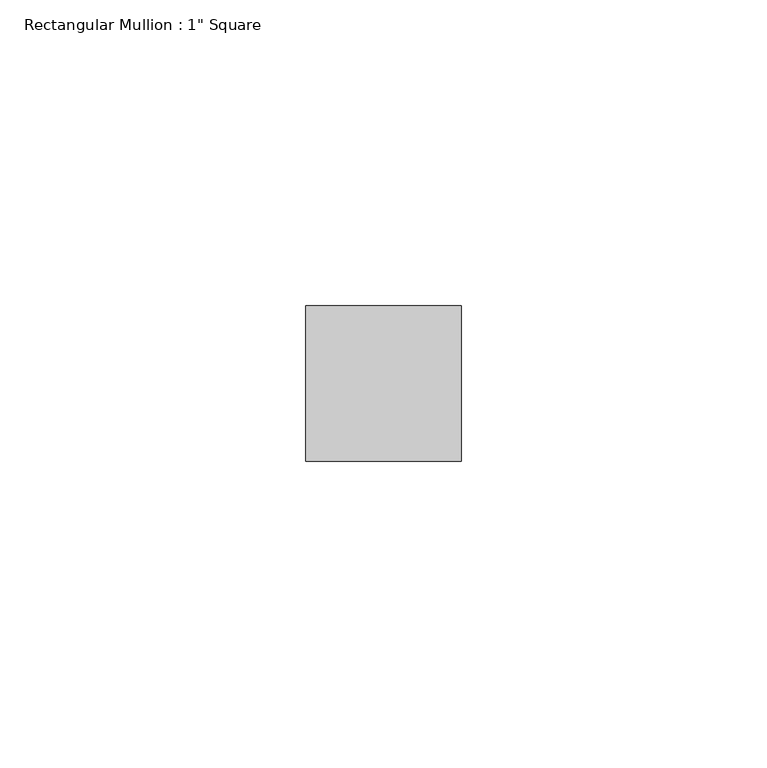
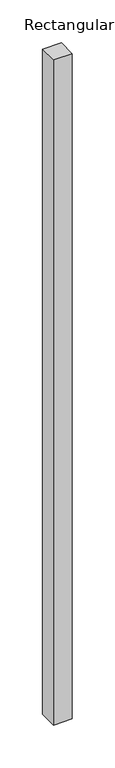
"""IFC4 building model written with IfcOpenShell, lengths in millimetres: member geometry."""

import ifcopenshell
import ifcopenshell.guid

model = None  # the IFC model being written
_history = None  # IfcOwnerHistory: only IFC2X3 demands one
_inside = {}  # id of a spatial element -> (the spatial element, [elements in it])
_under = {}  # id of a project, library or spatial element -> (it, [spatial elements below it])
_declared = {}  # id of a project -> (the project, [libraries it declares])
_typed = {}  # id of a type object -> (the type object, [elements of that type])
_made_of = {}  # id of a material, layer set ... -> (it, [elements and type objects made of it])


def new_model(schema):
    """Start an empty IFC model of exactly this schema.

    Asked for "IFC4X3", IfcOpenShell would pick the latest addendum, in which some entities
    have other attributes; the version numbers below select the first issue.
    IFC2X3 requires an IfcOwnerHistory on every rooted entity: one is made here for all.
    """
    global model, _history
    if schema == "IFC4X3":
        model = ifcopenshell.file(schema_version=(4, 3, 0, 0))
    else:
        model = ifcopenshell.file(schema=schema)
    _inside.clear()
    _under.clear()
    _declared.clear()
    _typed.clear()
    _made_of.clear()
    _history = None
    if model.schema == "IFC2X3":
        org = make("IfcOrganization", Name="unknown")
        user = make(
            "IfcPersonAndOrganization",
            ThePerson=make("IfcPerson", FamilyName="unknown"),
            TheOrganization=org,
        )
        app = make(
            "IfcApplication",
            ApplicationDeveloper=org,
            Version="unknown",
            ApplicationFullName="unknown",
            ApplicationIdentifier="unknown",
        )
        _history = make(
            "IfcOwnerHistory",
            OwningUser=user,
            OwningApplication=app,
            ChangeAction="ADDED",
            CreationDate=0,
        )
    return model


def make(cls, **values):
    """One entity of the class cls with the attributes given. An attribute that is None is left unset."""
    return model.create_entity(
        cls, **{name: value for name, value in values.items() if value is not None}
    )


def rooted(cls, **values):
    """An entity with a GlobalId (a new one), such as an element, a storey or a relation."""
    return make(cls, GlobalId=ifcopenshell.guid.new(), OwnerHistory=_history, **values)


def si_unit(unit_type, name, prefix=None):
    """IfcSIUnit, for example si_unit("LENGTHUNIT", "METRE", prefix="MILLI")."""
    return make("IfcSIUnit", UnitType=unit_type, Prefix=prefix, Name=name)


def assignment(units):
    """IfcUnitAssignment: the units of a project."""
    return None if units is None else make("IfcUnitAssignment", Units=units)


def point(xyz):
    """IfcCartesianPoint."""
    return None if xyz is None else make("IfcCartesianPoint", Coordinates=xyz)


def direction(xyz):
    """IfcDirection."""
    return None if xyz is None else make("IfcDirection", DirectionRatios=xyz)


def frame(location, z_axis=None, x_axis=None):
    """IfcAxis2Placement3D, a coordinate frame: its origin and axes. An axis left out is left unset."""
    return make(
        "IfcAxis2Placement3D",
        Location=point(location),
        Axis=direction(z_axis),
        RefDirection=direction(x_axis),
    )


def origin():
    """The frame at (0, 0, 0) with its axes left unset."""
    return frame((0.0, 0.0, 0.0))


def place(relative_to, where):
    """IfcLocalPlacement: puts the frame where relative to a parent placement (None: the world)."""
    return make(
        "IfcLocalPlacement", PlacementRelTo=relative_to, RelativePlacement=where
    )


def context(
    kind, dimensions, precision=None, world=None, true_north=None, identifier=None
):
    """IfcGeometricRepresentationContext, for example the 3D "Model" context."""
    return make(
        "IfcGeometricRepresentationContext",
        ContextIdentifier=identifier,
        ContextType=kind,
        CoordinateSpaceDimension=dimensions,
        Precision=precision,
        WorldCoordinateSystem=world,
        TrueNorth=true_north,
    )


def project(units=None, contexts=None):
    """IfcProject with its units and contexts."""
    return rooted(
        "IfcProject",
        Name="project",
        RepresentationContexts=contexts,
        UnitsInContext=assignment(units),
    )


def spatial(cls, under=None, at=None, **own):
    """A site, building, storey or space (cls), placed at a placement, below another one or the project."""
    s = rooted(cls, ObjectPlacement=at, **own)
    if under is not None:
        _under.setdefault(under.id(), (under, []))[1].append(s)
    return s


def polyline(points):
    """IfcPolyline through the points."""
    return make("IfcPolyline", Points=[point(p) for p in points])


def outline(outer, holes=None, kind="AREA"):
    """IfcArbitraryClosedProfileDef: a profile drawn as a closed curve; with holes, ...WithVoids."""
    if holes is None:
        return make("IfcArbitraryClosedProfileDef", ProfileType=kind, OuterCurve=outer)
    return make(
        "IfcArbitraryProfileDefWithVoids",
        ProfileType=kind,
        OuterCurve=outer,
        InnerCurves=holes,
    )


def extrude(swept, where, along, depth):
    """IfcExtrudedAreaSolid: the profile swept, set in the frame where, extruded along a direction by depth."""
    return make(
        "IfcExtrudedAreaSolid",
        SweptArea=swept,
        Position=where,
        ExtrudedDirection=direction(along),
        Depth=depth,
    )


def shape(context_of_items, identifier, shape_type, items):
    """IfcShapeRepresentation: the items that make up one representation, for example the "Body"."""
    return make(
        "IfcShapeRepresentation",
        ContextOfItems=context_of_items,
        RepresentationIdentifier=identifier,
        RepresentationType=shape_type,
        Items=items,
    )


def source(mapping_origin, context_of_items, identifier, shape_type, items):
    """IfcRepresentationMap: a shape defined once, which mapped items show again and again."""
    return make(
        "IfcRepresentationMap",
        MappingOrigin=mapping_origin,
        MappedRepresentation=shape(context_of_items, identifier, shape_type, items),
    )


def transform(
    local_origin,
    x_axis=None,
    y_axis=None,
    z_axis=None,
    scale=None,
    scale2=None,
    scale3=None,
    uniform=True,
):
    """IfcCartesianTransformationOperator3D, or its non-uniform kind. x_axis, y_axis, z_axis: its Axis1, 2, 3."""
    if uniform:
        return make(
            "IfcCartesianTransformationOperator3D",
            Axis1=direction(x_axis),
            Axis2=direction(y_axis),
            LocalOrigin=point(local_origin),
            Scale=scale,
            Axis3=direction(z_axis),
        )
    return make(
        "IfcCartesianTransformationOperator3DnonUniform",
        Axis1=direction(x_axis),
        Axis2=direction(y_axis),
        LocalOrigin=point(local_origin),
        Scale=scale,
        Axis3=direction(z_axis),
        Scale2=scale2,
        Scale3=scale3,
    )


def mapped(mapping_source, mapping_target):
    """IfcMappedItem: shows the shape of a source again, moved by a transform."""
    return make(
        "IfcMappedItem", MappingSource=mapping_source, MappingTarget=mapping_target
    )


def made_of(thing, what):
    """Note that an element or type object is made of a material, layer set ...; save() writes the relation."""
    if what is not None:
        _made_of.setdefault(what.id(), (what, []))[1].append(thing)
    return thing


def element(
    cls,
    number,
    at=None,
    inside=None,
    cuts=None,
    type_object=None,
    material=None,
    context=None,
    identifier="Body",
    shape_type=None,
    held_by="IfcProductDefinitionShape",
    body=None,
    shapes=None,
    **own,
):
    """One element of the class cls, such as IfcWall. Its Tag is "e" and its number.

    at: its placement. inside: the storey or other place that contains it. cuts: it is an
    opening in that element (IfcRelVoidsElement). A single representation is given by context,
    identifier, shape_type and body (its items); several are given by shapes. held_by: the class
    of the entity that holds the representations. save() writes the other relations.
    """
    e = rooted(cls, Tag="e%d" % number, ObjectPlacement=at, **own)
    if body is not None:
        shapes = [shape(context, identifier, shape_type, body)]
    if shapes is not None:
        e.Representation = make(held_by, Representations=shapes)
    if inside is not None:
        _inside.setdefault(inside.id(), (inside, []))[1].append(e)
    if cuts is not None:
        rooted(
            "IfcRelVoidsElement", RelatingBuildingElement=cuts, RelatedOpeningElement=e
        )
    if type_object is not None:
        _typed.setdefault(type_object.id(), (type_object, []))[1].append(e)
    return made_of(e, material)


def aggregate(whole, parts):
    """IfcRelAggregates: a whole, such as a stair, and the parts it consists of."""
    return rooted("IfcRelAggregates", RelatingObject=whole, RelatedObjects=parts)


def save(model, path):
    """Write the relations noted so far, then the file.

    IfcRelAggregates (storeys below a building ...), IfcRelContainedInSpatialStructure (elements
    in a storey), IfcRelDefinesByType, IfcRelAssociatesMaterial and IfcRelDeclares: one each for
    every whole, place, type object, material and project.
    """
    for whole, parts in _under.values():
        aggregate(whole, parts)
    for where, things in _inside.values():
        rooted(
            "IfcRelContainedInSpatialStructure",
            RelatedElements=things,
            RelatingStructure=where,
        )
    for kind, things in _typed.values():
        rooted("IfcRelDefinesByType", RelatedObjects=things, RelatingType=kind)
    for what, things in _made_of.values():
        rooted("IfcRelAssociatesMaterial", RelatedObjects=things, RelatingMaterial=what)
    for by, libraries in _declared.values():
        rooted("IfcRelDeclares", RelatingContext=by, RelatedDefinitions=libraries)
    model.write(path)


def member_867e3f91(model_context):
    return source(origin(), model_context, "Body", "SweptSolid", [
        extrude(outline(polyline([(12.7, 12.7), (12.7, -12.7), (-12.7, -12.7), (-12.7, 12.7), (12.7, 12.7)])), frame((0.0, 0.0, -949.4191728), z_axis=(0.0, 0.0, 1.0), x_axis=(1.0, 0.0, 0.0)), (0.0, 0.0, 1.0), 949.4191728),
    ])


if __name__ == "__main__":
    model = new_model("IFC4")
    model_context = context("Model", 3, world=origin())
    ifc_project = project(units=[si_unit("LENGTHUNIT", "METRE", prefix="MILLI")], contexts=[model_context])
    site = spatial("IfcSite", under=ifc_project)
    building = spatial("IfcBuilding", under=site)
    placement = place(None, origin())
    member_shape = member_867e3f91(model_context)
    element("IfcMember", 1, ObjectType="Rectangular Mullion : 1\" Square", at=placement, inside=building, context=model_context, shape_type="MappedRepresentation", body=[
        mapped(member_shape, transform((0.0, 0.0, 0.0), x_axis=(1.0, 0.0, 0.0), y_axis=(0.0, 1.0, 0.0), z_axis=(0.0, 0.0, 1.0))),
    ])
    save(model, "model.ifc")

# Revit data of these elements
# Type "Rectangular Mullion : 1\" Square"
#   built-in parameter 1007304 = 0.0833333 (stored number, unit not read)
#   built-in parameter 1007301 = 0.0416667 (stored number, unit not read)
#   built-in parameter 1007300 = 0.0416667 (stored number, unit not read)
# Element 1 (IfcMember, "Rectangular Mullion : 1\" Square")
#   Materials on its faces: "Metal - Aluminum"
# Materials
#   "Metal - Aluminum": class "Metal", colour RGB 247 247 247, transparency 0
